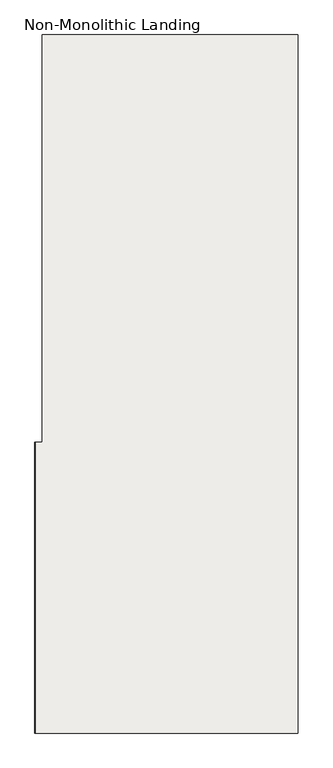
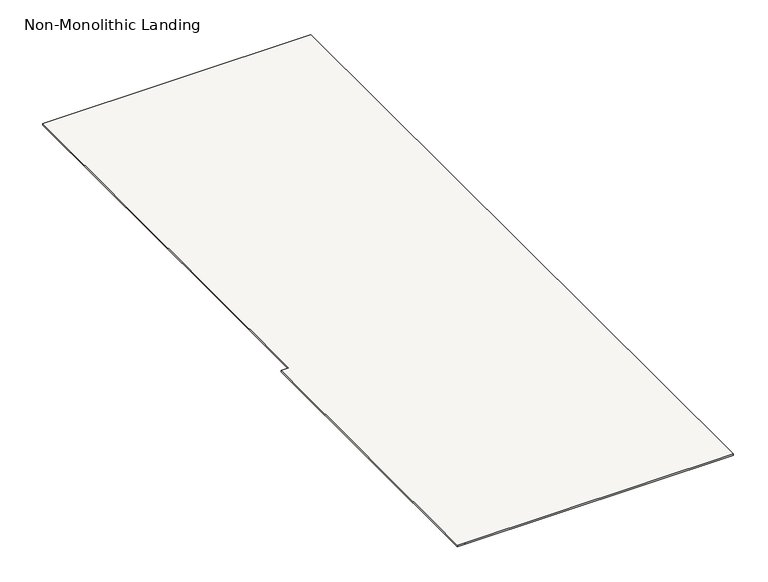
"""IFC4 building model written with IfcOpenShell, lengths in millimetres: slab geometry, Non-Monolithic Landing."""

from ifc_helpers import new_model, si_unit, origin, place, context, project, spatial, faceted_brep, source, transform, mapped, element, save


def non_monolithic_landing_bae31da9(model_context):
    return source(origin(), model_context, "Body", "Brep", [
        faceted_brep([(-13356.0599092, 11470.4345331, 16294.1176471), (-13356.9099092, 11470.4345331, 16288.1176471), (-13356.9099092, 10220.4345331, 16288.1176471), (-13356.0599092, 10220.4345331, 16294.1176471), (-13325.0, 12030.4345331, 16294.1176471), (-13325.0, 11470.4345331, 16294.1176471), (-13325.0, 10220.4345331, 16294.1176471), (-12225.0, 10220.4345331, 16294.1176471), (-12225.0, 13220.4345331, 16294.1176471), (-13325.0, 13220.4345331, 16294.1176471), (-13325.0, 11470.4345331, 16288.1176471), (-13325.0, 12030.4345331, 16288.1176471), (-13324.15, 12030.4345331, 16288.1176471), (-13324.15, 13220.4345331, 16288.1176471), (-12225.0, 13220.4345331, 16288.1176471), (-12225.0, 10220.4345331, 16288.1176471), (-13325.0, 10220.4345331, 16288.1176471)], [[[0, 1, 2, 3]], [[4, 5, 0, 3, 6, 7, 8, 9]], [[10, 11, 12, 13, 14, 15, 16, 2, 1]], [[5, 4, 11, 10]], [[0, 5, 10, 1]], [[6, 3, 2, 16]], [[7, 6, 16, 15]], [[8, 7, 15, 14]], [[9, 8, 14, 13]], [[4, 12, 11]], [[12, 4, 9, 13]]]),
    ])


if __name__ == "__main__":
    model = new_model("IFC4")
    model_context = context("Model", 3, world=origin())
    ifc_project = project(units=[si_unit("LENGTHUNIT", "METRE", prefix="MILLI")], contexts=[model_context])
    site = spatial("IfcSite", under=ifc_project)
    building = spatial("IfcBuilding", under=site)
    placement = place(None, origin())
    non_monolithic_landing_shape = non_monolithic_landing_bae31da9(model_context)
    element("IfcSlab", 1, ObjectType="Non-Monolithic Landing", at=placement, inside=building, context=model_context, shape_type="MappedRepresentation", body=[
        mapped(non_monolithic_landing_shape, transform((0.0, 0.0, 0.0), x_axis=(1.0, 0.0, 0.0), y_axis=(0.0, 1.0, 0.0), z_axis=(0.0, 0.0, 1.0))),
    ])
    save(model, "model.ifc")

# Revit data of these elements
# Element 1 (IfcSlab, "Non-Monolithic Landing")
#   Materials on its faces: "Steel, Paint Finish, Dark Gray"
# Materials
#   "Steel, Paint Finish, Dark Gray": class "Metal", colour RGB 89 89 89, transparency 0, Description = "Steel, paint finish, dark gray, glossy", Cost = 0
